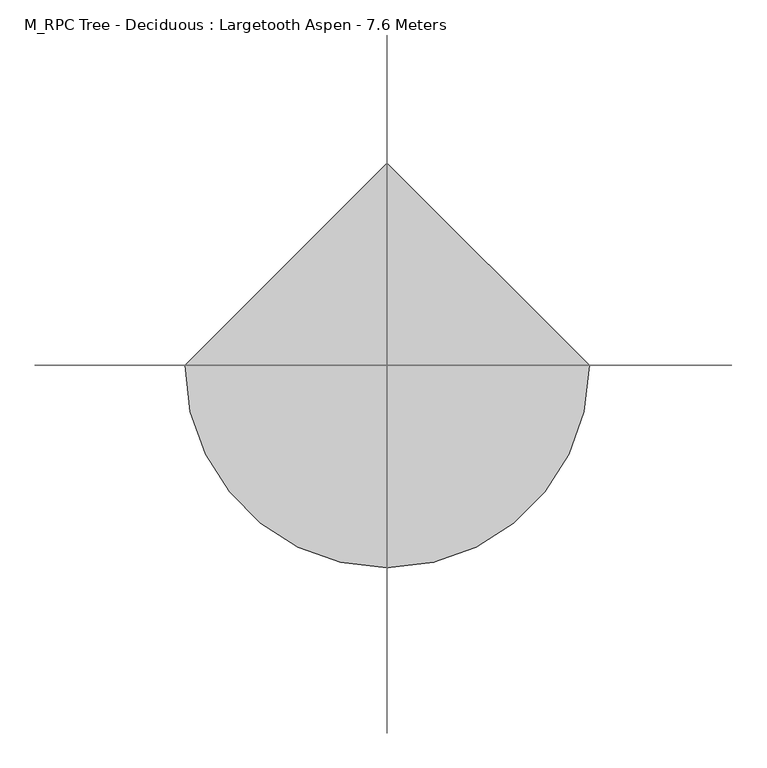
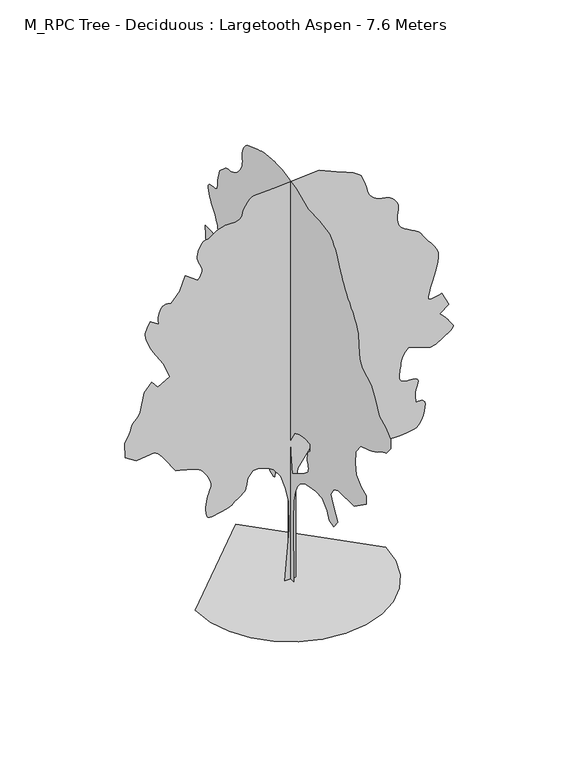
"""IFC4 building model written with IfcOpenShell, lengths in millimetres: geographic element geometry, M_RPC Tree - Deciduous : Largetooth Aspen - 7.6 Meters."""

import ifcopenshell
import ifcopenshell.guid

model = None  # the IFC model being written
_history = None  # IfcOwnerHistory: only IFC2X3 demands one
_inside = {}  # id of a spatial element -> (the spatial element, [elements in it])
_under = {}  # id of a project, library or spatial element -> (it, [spatial elements below it])
_declared = {}  # id of a project -> (the project, [libraries it declares])
_typed = {}  # id of a type object -> (the type object, [elements of that type])
_made_of = {}  # id of a material, layer set ... -> (it, [elements and type objects made of it])


def new_model(schema):
    """Start an empty IFC model of exactly this schema.

    Asked for "IFC4X3", IfcOpenShell would pick the latest addendum, in which some entities
    have other attributes; the version numbers below select the first issue.
    IFC2X3 requires an IfcOwnerHistory on every rooted entity: one is made here for all.
    """
    global model, _history
    if schema == "IFC4X3":
        model = ifcopenshell.file(schema_version=(4, 3, 0, 0))
    else:
        model = ifcopenshell.file(schema=schema)
    _inside.clear()
    _under.clear()
    _declared.clear()
    _typed.clear()
    _made_of.clear()
    _history = None
    if model.schema == "IFC2X3":
        org = make("IfcOrganization", Name="unknown")
        user = make(
            "IfcPersonAndOrganization",
            ThePerson=make("IfcPerson", FamilyName="unknown"),
            TheOrganization=org,
        )
        app = make(
            "IfcApplication",
            ApplicationDeveloper=org,
            Version="unknown",
            ApplicationFullName="unknown",
            ApplicationIdentifier="unknown",
        )
        _history = make(
            "IfcOwnerHistory",
            OwningUser=user,
            OwningApplication=app,
            ChangeAction="ADDED",
            CreationDate=0,
        )
    return model


def make(cls, **values):
    """One entity of the class cls with the attributes given. An attribute that is None is left unset."""
    return model.create_entity(
        cls, **{name: value for name, value in values.items() if value is not None}
    )


def rooted(cls, **values):
    """An entity with a GlobalId (a new one), such as an element, a storey or a relation."""
    return make(cls, GlobalId=ifcopenshell.guid.new(), OwnerHistory=_history, **values)


def si_unit(unit_type, name, prefix=None):
    """IfcSIUnit, for example si_unit("LENGTHUNIT", "METRE", prefix="MILLI")."""
    return make("IfcSIUnit", UnitType=unit_type, Prefix=prefix, Name=name)


def assignment(units):
    """IfcUnitAssignment: the units of a project."""
    return None if units is None else make("IfcUnitAssignment", Units=units)


def point(xyz):
    """IfcCartesianPoint."""
    return None if xyz is None else make("IfcCartesianPoint", Coordinates=xyz)


def direction(xyz):
    """IfcDirection."""
    return None if xyz is None else make("IfcDirection", DirectionRatios=xyz)


def frame(location, z_axis=None, x_axis=None):
    """IfcAxis2Placement3D, a coordinate frame: its origin and axes. An axis left out is left unset."""
    return make(
        "IfcAxis2Placement3D",
        Location=point(location),
        Axis=direction(z_axis),
        RefDirection=direction(x_axis),
    )


def origin():
    """The frame at (0, 0, 0) with its axes left unset."""
    return frame((0.0, 0.0, 0.0))


def place(relative_to, where):
    """IfcLocalPlacement: puts the frame where relative to a parent placement (None: the world)."""
    return make(
        "IfcLocalPlacement", PlacementRelTo=relative_to, RelativePlacement=where
    )


def context(
    kind, dimensions, precision=None, world=None, true_north=None, identifier=None
):
    """IfcGeometricRepresentationContext, for example the 3D "Model" context."""
    return make(
        "IfcGeometricRepresentationContext",
        ContextIdentifier=identifier,
        ContextType=kind,
        CoordinateSpaceDimension=dimensions,
        Precision=precision,
        WorldCoordinateSystem=world,
        TrueNorth=true_north,
    )


def project(units=None, contexts=None):
    """IfcProject with its units and contexts."""
    return rooted(
        "IfcProject",
        Name="project",
        RepresentationContexts=contexts,
        UnitsInContext=assignment(units),
    )


def spatial(cls, under=None, at=None, **own):
    """A site, building, storey or space (cls), placed at a placement, below another one or the project."""
    s = rooted(cls, ObjectPlacement=at, **own)
    if under is not None:
        _under.setdefault(under.id(), (under, []))[1].append(s)
    return s


def point_list(points):
    """IfcCartesianPointList2D or 3D."""
    cls = (
        "IfcCartesianPointList2D" if len(points[0]) == 2 else "IfcCartesianPointList3D"
    )
    return make(cls, CoordList=points)


def triangles(points, corners, closed=None, point_numbers=None):
    """IfcTriangulatedFaceSet: each triangle names its three corners, points numbered from 1."""
    return make(
        "IfcTriangulatedFaceSet",
        Coordinates=point_list(points),
        Closed=closed,
        CoordIndex=corners,
        PnIndex=point_numbers,
    )


def shape(context_of_items, identifier, shape_type, items):
    """IfcShapeRepresentation: the items that make up one representation, for example the "Body"."""
    return make(
        "IfcShapeRepresentation",
        ContextOfItems=context_of_items,
        RepresentationIdentifier=identifier,
        RepresentationType=shape_type,
        Items=items,
    )


def source(mapping_origin, context_of_items, identifier, shape_type, items):
    """IfcRepresentationMap: a shape defined once, which mapped items show again and again."""
    return make(
        "IfcRepresentationMap",
        MappingOrigin=mapping_origin,
        MappedRepresentation=shape(context_of_items, identifier, shape_type, items),
    )


def transform(
    local_origin,
    x_axis=None,
    y_axis=None,
    z_axis=None,
    scale=None,
    scale2=None,
    scale3=None,
    uniform=True,
):
    """IfcCartesianTransformationOperator3D, or its non-uniform kind. x_axis, y_axis, z_axis: its Axis1, 2, 3."""
    if uniform:
        return make(
            "IfcCartesianTransformationOperator3D",
            Axis1=direction(x_axis),
            Axis2=direction(y_axis),
            LocalOrigin=point(local_origin),
            Scale=scale,
            Axis3=direction(z_axis),
        )
    return make(
        "IfcCartesianTransformationOperator3DnonUniform",
        Axis1=direction(x_axis),
        Axis2=direction(y_axis),
        LocalOrigin=point(local_origin),
        Scale=scale,
        Axis3=direction(z_axis),
        Scale2=scale2,
        Scale3=scale3,
    )


def mapped(mapping_source, mapping_target):
    """IfcMappedItem: shows the shape of a source again, moved by a transform."""
    return make(
        "IfcMappedItem", MappingSource=mapping_source, MappingTarget=mapping_target
    )


def made_of(thing, what):
    """Note that an element or type object is made of a material, layer set ...; save() writes the relation."""
    if what is not None:
        _made_of.setdefault(what.id(), (what, []))[1].append(thing)
    return thing


def element(
    cls,
    number,
    at=None,
    inside=None,
    cuts=None,
    type_object=None,
    material=None,
    context=None,
    identifier="Body",
    shape_type=None,
    held_by="IfcProductDefinitionShape",
    body=None,
    shapes=None,
    **own,
):
    """One element of the class cls, such as IfcWall. Its Tag is "e" and its number.

    at: its placement. inside: the storey or other place that contains it. cuts: it is an
    opening in that element (IfcRelVoidsElement). A single representation is given by context,
    identifier, shape_type and body (its items); several are given by shapes. held_by: the class
    of the entity that holds the representations. save() writes the other relations.
    """
    e = rooted(cls, Tag="e%d" % number, ObjectPlacement=at, **own)
    if body is not None:
        shapes = [shape(context, identifier, shape_type, body)]
    if shapes is not None:
        e.Representation = make(held_by, Representations=shapes)
    if inside is not None:
        _inside.setdefault(inside.id(), (inside, []))[1].append(e)
    if cuts is not None:
        rooted(
            "IfcRelVoidsElement", RelatingBuildingElement=cuts, RelatedOpeningElement=e
        )
    if type_object is not None:
        _typed.setdefault(type_object.id(), (type_object, []))[1].append(e)
    return made_of(e, material)


def aggregate(whole, parts):
    """IfcRelAggregates: a whole, such as a stair, and the parts it consists of."""
    return rooted("IfcRelAggregates", RelatingObject=whole, RelatedObjects=parts)


def save(model, path):
    """Write the relations noted so far, then the file.

    IfcRelAggregates (storeys below a building ...), IfcRelContainedInSpatialStructure (elements
    in a storey), IfcRelDefinesByType, IfcRelAssociatesMaterial and IfcRelDeclares: one each for
    every whole, place, type object, material and project.
    """
    for whole, parts in _under.values():
        aggregate(whole, parts)
    for where, things in _inside.values():
        rooted(
            "IfcRelContainedInSpatialStructure",
            RelatedElements=things,
            RelatingStructure=where,
        )
    for kind, things in _typed.values():
        rooted("IfcRelDefinesByType", RelatedObjects=things, RelatingType=kind)
    for what, things in _made_of.values():
        rooted("IfcRelAssociatesMaterial", RelatedObjects=things, RelatingMaterial=what)
    for by, libraries in _declared.values():
        rooted("IfcRelDeclares", RelatingContext=by, RelatedDefinitions=libraries)
    model.write(path)


def m_rpc_tree_deciduous_largetooth_aspen_7_6_meters_7a32e79d(model_context):
    return source(origin(), model_context, "Body", "Tessellation", [
        triangles([(92.8617737, 0.000406, 0.005513), (-103.915959, 0.000406, 0.005513), (-22.8901635, 0.0003494, 949.168154), (-34.4652064, 0.0003176, 1481.626133), (-92.3406663, 0.0003011, 1759.4311237), (-173.3674883, 0.0002866, 2002.5093098), (-300.6937099, 0.0002762, 2176.1362118), (-404.8693279, 0.0002728, 2234.0127663), (-566.9214277, 0.0002694, 2291.8891754), (-682.6743914, 0.0002694, 2291.8891754), (-763.7004776, 0.0002762, 2176.1362118), (-798.427355, 0.0002852, 2025.6589142), (-801.2950579, 0.0002863, 2008.1460297), (-806.4934324, 0.0002874, 1989.7185207), (-816.3455927, 0.0002886, 1969.4722275), (-833.1871519, 0.0002899, 1946.489764), (-859.3387533, 0.0002915, 1919.8644997), (-897.1360102, 0.0002934, 1888.6816647), (-948.9046526, 0.0002956, 1852.0320122), (-998.3097038, 0.0002977, 1817.003627), (-1032.3247061, 0.0002993, 1790.0718407), (-1058.2431822, 0.0003005, 1769.4200489), (-1083.3510246, 0.0003015, 1753.2220551), (-1114.9365967, 0.0003023, 1739.6560226), (-1160.2933485, 0.000303, 1726.8980804), (-1226.7072453, 0.0003038, 1713.1294441), (-1299.8367931, 0.0003048, 1697.5064152), (-1361.0192505, 0.0003056, 1683.0943588), (-1411.0653236, 0.0003062, 1673.9516029), (-1450.7854282, 0.0003062, 1674.1187439), (-1480.9902706, 0.0003054, 1687.6517841), (-1502.4856155, 0.0003035, 1718.5964069), (-1516.0869656, 0.0003004, 1771.0059986), (-1522.0251205, 0.0002967, 1833.4045155), (-1521.0802654, 0.0002932, 1891.7521168), (-1514.8710514, 0.00029, 1946.2541679), (-1505.0164204, 0.0002869, 1997.1108021), (-1493.1376396, 0.0002841, 2044.5246231), (-1480.8535057, 0.0002815, 2088.6983803), (-1469.7852859, 0.000279, 2129.8371483), (-1458.1775642, 0.0002769, 2165.8103886), (-1444.9485752, 0.000275, 2196.5194153), (-1432.7328964, 0.0002733, 2225.2042923), (-1424.1600185, 0.0002715, 2255.1052288), (-1421.8648098, 0.0002695, 2289.4596725), (-1428.479377, 0.000267, 2331.5079781), (-1446.6358269, 0.0002638, 2384.4900639), (-1473.3978561, 0.0002604, 2441.7913628), (-1503.3976238, 0.0002573, 2494.2338013), (-1535.6266159, 0.0002545, 2541.2094223), (-1569.0690514, 0.0002521, 2582.1229134), (-1602.7142361, 0.00025, 2616.3228607), (-1635.5487144, 0.0002484, 2643.2520309), (-1666.5644085, 0.0002473, 2662.3026123), (-1701.7269424, 0.0002464, 2677.1732162), (-1746.6125748, 0.0002455, 2692.0694), (-1799.5946606, 0.0002446, 2706.940004), (-1859.0570194, 0.0002437, 2721.8358971), (-1923.3782387, 0.0002428, 2736.706501), (-1990.9396671, 0.000242, 2751.5773956), (-2060.1198921, 0.0002411, 2766.4732887), (-2256.8962532, 0.0002238, 3055.8556252), (-2301.7818855, 0.0002202, 3116.5289566), (-2338.160479, 0.0002175, 3161.4195305), (-2367.4508423, 0.0002156, 3193.1367805), (-2391.0741096, 0.0002144, 3214.3154297), (-2410.4440029, 0.0002136, 3227.61549), (-2426.9816563, 0.0002131, 3235.6461044), (-2442.1006462, 0.0002128, 3241.041996), (-2766.1945267, 0.0002148, 3206.3353935), (-2962.9836777, 0.0002073, 3333.6607613), (-2974.5611687, 0.0001914, 3599.8884064), (-2952.3436295, 0.000189, 3639.5351143), (-2930.8612198, 0.0001867, 3678.9789276), (-2910.7717484, 0.0001843, 3718.0431129), (-2892.8103447, 0.0001821, 3756.473616), (-2877.7118477, 0.0001798, 3794.0937035), (-2866.1343567, 0.0001776, 3830.70019), (-2858.8132919, 0.0001755, 3866.1160515), (-2847.3878265, 0.0001735, 3899.5814507), (-2825.6772331, 0.0001716, 3931.2481224), (-2797.4559906, 0.0001698, 3962.0787987), (-2766.6000252, 0.0001679, 3993.137368), (-2736.9852631, 0.000166, 4025.3865623), (-2712.4120537, 0.000164, 4059.8905609), (-2696.7560326, 0.0001617, 4097.611805), (-2627.2919586, 0.000141, 4444.881015), (-2488.4021805, 0.0001321, 4595.3354942), (-2384.2240917, 0.0001396, 4468.0101265), (-2164.2955101, 0.0001327, 4583.7835831), (-2280.0484737, 0.0001155, 4873.1406303), (-2465.2501053, 9.82e-05, 5162.5226761), (-2487.5231644, 9.58e-05, 5203.6643509), (-2513.0364326, 9.27e-05, 5254.9385468), (-2539.3601166, 8.93e-05, 5312.268187), (-2564.0600624, 8.58e-05, 5371.6238663), (-2584.7067673, 8.24e-05, 5428.9535065), (-2598.8934013, 7.93e-05, 5480.2277023), (-2604.1628471, 7.69e-05, 5521.3693771), (-2601.4519661, 7.48e-05, 5555.7463486), (-2593.9027176, 7.28e-05, 5589.5413788), (-2582.2746483, 7.08e-05, 5622.8038834), (-2567.4293335, 6.89e-05, 5655.6611801), (-2550.1521904, 6.69e-05, 5688.2394241), (-2531.2585762, 6.5e-05, 5720.5903564), (-2511.5516396, 6.31e-05, 5752.8651306), (-2361.0744873, 6.93e-05, 5648.6941635), (-2365.8675087, 6.73e-05, 5681.019516), (-2369.6472198, 6.54e-05, 5713.8518143), (-2371.4003105, 6.34e-05, 5747.6968414), (-2370.118412, 6.13e-05, 5783.0621246), (-2364.7857433, 5.9e-05, 5820.4540283), (-2354.391465, 5.67e-05, 5860.3794983), (-2337.9248829, 5.41e-05, 5903.344899), (-2316.394075, 5.19e-05, 5940.9141174), (-2291.8258072, 5.04e-05, 5965.7155106), (-2264.7268799, 4.95e-05, 5979.8768555), (-2235.6036575, 4.92e-05, 5985.5515091), (-2204.9604698, 4.92e-05, 5984.8422501), (-2173.3064426, 4.95e-05, 5979.8768555), (-2141.1459057, 5e-05, 5972.7836838), (-1990.6686081, 3.96e-05, 6146.4178528), (-1886.4929901, 2.44e-05, 6401.0685883), (-1666.5644085, 3.41e-05, 6239.0110382), (-1644.4939533, 3.23e-05, 6268.8284042), (-1623.9409927, 3.05e-05, 6298.823085), (-1606.4256374, 2.87e-05, 6329.2229736), (-1593.4675621, 2.69e-05, 6360.2309647), (-1586.584552, 2.5e-05, 6392.0749512), (-1587.2913403, 2.3e-05, 6424.9066681), (-1597.1131245, 2.1e-05, 6458.9551712), (-1613.1085144, 1.89e-05, 6493.7885101), (-1630.1173599, 1.68e-05, 6529.2043716), (-1646.3154991, 1.46e-05, 6565.8614365), (-1659.8813862, 1.23e-05, 6604.3428085), (-1668.993766, 9.9e-06, 6645.2310104), (-1671.8286221, 7.3e-06, 6689.1585617), (-1666.5644085, 4.4e-06, 6736.759726), (-1653.9432312, 1.5e-06, 6785.3747818), (-1636.4607227, -1.2e-06, 6830.974324), (-1614.9300602, -3.6e-06, 6871.9131042), (-1590.1616592, -5.7e-06, 6906.5691284), (-1562.9612846, -7.3e-06, 6933.3209839), (-1534.1394974, -8.3e-06, 6950.5728378), (-1504.512236, -8.7e-06, 6956.6782791), (-1471.3382435, -9.2e-06, 6965.0132355), (-1431.8891979, -1.05e-05, 6986.521225), (-1386.9707188, -1.22e-05, 7015.9078033), (-1337.3959831, -1.41e-05, 7047.9291046), (-1283.9756973, -1.59e-05, 7077.315683), (-1227.5178062, -1.72e-05, 7098.8236725), (-1168.8306908, -1.77e-05, 7107.1580475), (-1109.0314339, -1.76e-05, 7106.8289978), (-1050.4481638, -1.77e-05, 7107.2847839), (-995.7104439, -1.79e-05, 7110.8060806), (-947.4530697, -1.84e-05, 7119.5718246), (-908.3055319, -1.94e-05, 7135.8353668), (-880.9024807, -2.09e-05, 7161.8273849), (-867.8760956, -2.32e-05, 7199.7512329), (-856.9422426, -2.61e-05, 7248.5941818), (-835.6824938, -2.93e-05, 7302.6809967), (-806.5264246, -3.26e-05, 7357.4009125), (-771.9008492, -3.56e-05, 7408.0420074), (-734.2403572, -3.81e-05, 7449.9940979), (-695.9718355, -3.98e-05, 7478.5696793), (-659.5247869, -4.04e-05, 7489.1341507), (-323.8458215, -4.18e-05, 7512.2885513), (509.5693688, -4.53e-05, 7570.1751343), (926.2744205, -3.42e-05, 7384.9631836), (995.3532709, -3.26e-05, 7357.5526474), (1062.2079111, -3.09e-05, 7329.4578506), (1124.6038118, -2.92e-05, 7299.9195374), (1180.3219225, -2.73e-05, 7268.2778641), (1227.1277138, -2.52e-05, 7233.7741562), (1262.7970482, -2.29e-05, 7195.7485703), (1285.1055702, -2.04e-05, 7153.4674301), (1299.9533558, -1.79e-05, 7111.9461273), (1314.5985374, -1.58e-05, 7075.1117477), (1328.8409821, -1.37e-05, 7040.4813034), (1342.4753242, -1.16e-05, 7005.6479645), (1355.2991055, -9.4e-06, 6968.1799026), (1367.1094311, -6.8e-06, 6925.6702881), (1377.7063133, -3.9e-06, 6875.662294), (1393.5345623, -8e-07, 6823.9573105), (1419.2834267, 2e-06, 6778.1292938), (1452.117905, 4.3e-06, 6738.3811386), (1489.2059029, 6.3e-06, 6704.890741), (1527.709948, 7.9e-06, 6677.9109924), (1564.7979458, 9.1e-06, 6657.5936279), (1597.6348949, 9.9e-06, 6644.1415421), (1628.0070236, 1.04e-05, 6636.0856384), (1659.1872425, 1.07e-05, 6630.6638763), (1690.5726814, 1.1e-05, 6626.2310074), (1721.5527672, 1.13e-05, 6621.2150345), (1751.5195427, 1.17e-05, 6613.9439667), (1779.8675217, 1.24e-05, 6602.8481323), (1805.9862762, 1.34e-05, 6586.2799576), (1831.2638031, 1.47e-05, 6563.7586578), (1856.5388592, 1.63e-05, 6536.6015945), (1880.3977226, 1.82e-05, 6505.7964981), (1901.4218754, 2.02e-05, 6472.3560974), (1918.1949795, 2.23e-05, 6437.2948654), (1929.2986622, 2.44e-05, 6401.625531), (1933.3139694, 2.65e-05, 6366.3364059), (1929.8053173, 2.9e-05, 6325.1191544), (1922.245895, 3.2e-05, 6273.1351181), (1915.0916805, 3.56e-05, 6213.8805954), (1912.7964718, 3.93e-05, 6150.775145), (1919.8163921, 4.31e-05, 6087.2644867), (1940.6048035, 4.67e-05, 6026.7937592), (1979.615649, 5e-05, 5972.7836838), (2034.2165314, 5.26e-05, 5927.5631882), (2096.1082478, 5.5e-05, 5888.8289246), (2161.2403187, 5.71e-05, 5853.1340103), (2225.5615379, 5.92e-05, 5817.0088898), (2285.0238968, 6.16e-05, 5777.0584213), (2335.5764797, 6.44e-05, 5729.8118866), (2373.1711327, 6.79e-05, 5671.8491455), (2411.6423309, 7.17e-05, 5607.2240204), (2462.6659607, 7.56e-05, 5541.7878983), (2518.9567108, 7.96e-05, 5474.7303635), (2573.2307236, 8.38e-05, 5405.2415817), (2618.1721664, 8.81e-05, 5332.5093933), (2646.5201454, 9.27e-05, 5255.7495438), (2650.9785942, 9.76e-05, 5174.1004578), (2634.6386032, 0.0001032, 5079.7841217), (2608.190799, 0.0001097, 4970.8762344), (2575.6628426, 0.0001165, 4855.508567), (2541.0826859, 0.0001233, 4741.7367325), (2508.5625778, 0.0001295, 4637.6927925), (2482.1043091, 0.0001347, 4551.4835197), (2465.7718758, 0.0001383, 4491.1648178), (2464.9611694, 0.0001404, 4454.9635391), (2480.5538223, 0.0001417, 4433.9369156), (2509.8113388, 0.0001422, 4425.5769608), (2550.0001648, 0.0001421, 4427.3248192), (2598.3867462, 0.0001415, 4436.6727951), (2652.2453773, 0.0001407, 4451.0876129), (2708.839888, 0.0001396, 4468.0101265), (2836.1652557, 0.0001548, 4213.3596817), (2674.1332855, 0.0001624, 4086.0346046), (2698.8841003, 0.0001637, 4063.6400414), (2723.4573097, 0.0001651, 4040.7132431), (2747.6253113, 0.0001665, 4016.7987144), (2771.1852104, 0.0001681, 3991.3386406), (2793.9346939, 0.0001697, 3963.8775261), (2815.6705765, 0.0001715, 3933.8828453), (2836.1652557, 0.0001735, 3900.8482338), (2858.1037422, 0.0001754, 3868.6749069), (2881.2584335, 0.000177, 3840.554821), (2901.1705902, 0.0001786, 3814.8921432), (2913.3811821, 0.0001801, 3790.0148827), (2913.4570496, 0.0001816, 3764.3269157), (2896.9144547, 0.0001833, 3736.2324097), (2859.3199471, 0.0001852, 3704.0590828), (2604.6695023, 0.0001955, 3530.4246231), (2500.4962097, 0.0001962, 3518.8471321), (2118.5182171, 0.0001886, 3646.1724998), (2091.3836815, 0.0001903, 3618.7110947), (2065.163625, 0.000192, 3590.1352226), (2040.7651142, 0.0001938, 3559.3298355), (2019.0975414, 0.0001958, 3525.1551773), (2001.0780018, 0.0001981, 3486.5726486), (1987.6134167, 0.0002008, 3442.3913338), (1979.615649, 0.0002038, 3391.5220551), (1974.0473843, 0.0002068, 3342.1474525), (1967.6684132, 0.0002092, 3301.2848305), (1961.0868382, 0.0002113, 3266.096862), (1954.9106163, 0.0002132, 3233.7209312), (1949.7477047, 0.0002151, 3201.3702896), (1946.2035896, 0.0002172, 3166.1567413), (1944.888699, 0.0002197, 3125.2941193), (1953.8643139, 0.000222, 3086.7368797), (1977.0163891, 0.0002236, 3059.0981598), (2008.6704163, 0.0002247, 3040.5542336), (2043.1591541, 0.0002254, 3029.3316628), (2074.8131813, 0.0002257, 3023.5555618), (2097.9652565, 0.0002259, 3021.4277847), (2106.9408714, 0.0002259, 3021.1237335), (2119.5973663, 0.0002258, 3022.0103073), (2151.4869896, 0.0002258, 3022.4663841), (2193.5021576, 0.000226, 3019.2997169), (2236.5307812, 0.0002266, 3009.242482), (2271.4578644, 0.0002278, 2989.0771431), (2289.1759689, 0.0002298, 2955.5102966), (2280.5702442, 0.0002328, 2905.3758568), (2259.8146797, 0.0002362, 2847.8691925), (2246.3500946, 0.0002394, 2794.0105614), (2238.9578133, 0.0002425, 2743.191861), (2236.4270084, 0.0002453, 2694.7799904), (2237.5416206, 0.0002481, 2648.2174255), (2241.0857357, 0.0002508, 2602.8707748), (2245.8434395, 0.0002535, 2558.1069374), (2285.1910378, 0.0002532, 2562.540097), (2322.5171024, 0.0002531, 2563.730722), (2355.7899261, 0.0002535, 2558.4106979), (2382.9903008, 0.0002544, 2543.4133575), (2402.0916058, 0.000256, 2515.4278564), (2411.0672207, 0.0002587, 2471.2540993), (2407.8954666, 0.0002625, 2407.6396683), (2395.1731327, 0.0002668, 2334.9507912), (2376.983836, 0.0002708, 2266.9155544), (2353.5301804, 0.0002745, 2205.3632069), (2325.0124443, 0.0002777, 2152.110062), (2291.638464, 0.0002803, 2108.9801365), (2253.6054657, 0.0002821, 2077.7999176), (2211.1189602, 0.0002832, 2060.3858643), (2171.2620907, 0.0002837, 2051.7801395), (2137.4826118, 0.000284, 2045.4011684), (2104.5113686, 0.0002843, 2040.64361), (2067.0864727, 0.0002845, 2036.8967457), (2019.9412399, 0.0002847, 2033.5578506), (1957.8137821, 0.000285, 2030.0137356), (1875.4374149, 0.0002852, 2025.6589142), (1785.9069786, 0.0002851, 2027.1105698), (1704.880965, 0.0002844, 2040.1039627), (1630.9407108, 0.000283, 2062.7139198), (1562.6724941, 0.0002812, 2093.0175934), (1498.6551807, 0.0002791, 2129.0947517), (1437.4727234, 0.0002767, 2169.0176056), (1377.7063133, 0.0002742, 2210.8631618), (1123.0508543, 0.0002597, 2453.9412025), (856.8231365, 0.0002528, 2569.6841377), (544.2937391, 0.0002542, 2546.5547356), (393.8164052, 0.0002611, 2430.7917435), (289.6407872, 0.00027, 2280.3144459), (127.5871523, 0.0002838, 2048.8109894), (92.8617737, 0.0003011, 1759.4311237), (92.8617737, 0.0003383, 1134.3723289), (-0.0023646, 90.6053344, 1.1e-05), (-0.0023646, -94.5971056, 0.0), (-0.0023646, -83.0220672, 1157.5168465), (-0.0023646, -94.5971056, 1527.9227257), (-0.0023646, -140.8980313, 1724.6992321), (-0.0023646, -210.3490428, 1875.1765297), (-0.0023646, -302.9508941, 1990.9294933), (-0.0023646, -441.853444, 2071.9555069), (-0.0023646, -557.6038642, 2095.1051113), (-0.0023646, -789.1072117, 2141.4067909), (-0.0023646, -985.8861889, 2129.8320614), (-0.0023646, -1136.3635592, 1979.3547638), (-0.0023646, -1205.8147705, 1840.4521957), (-0.0023646, -1333.1399929, 1794.1505161), (-0.0023646, -1472.042561, 1967.7774181), (-0.0023646, -1321.5652634, 2199.2833454), (-0.0023646, -1252.1139793, 2361.3353725), (-0.0023646, -1333.1399929, 2500.2354698), (-0.0023646, -1483.6172905, 2569.6841377), (-0.0023646, -1969.7736626, 2569.6841377), (-0.0023646, -2351.7542713, 2835.9117828), (-0.0023646, -2351.7542713, 2997.9690422), (-0.0023646, -2189.7022442, 3067.4075363), (-0.0023646, -2039.2249466, 3206.3101044), (-0.0023646, -2004.5006126, 3403.0992554), (-0.0023646, -2027.6500717, 3634.5950089), (-0.0023646, -2178.1273693, 3831.3841599), (-0.0023646, -2444.3551598, 3923.9773453), (-0.0023646, -2488.9367409, 3941.4068047), (-0.0023646, -2533.110498, 3959.1147354), (-0.0023646, -2576.4735489, 3977.4307686), (-0.0023646, -2618.6279526, 3996.6839539), (-0.0023646, -2659.1612343, 4017.1280548), (-0.0023646, -2697.6678955, 4039.0921211), (-0.0023646, -2733.7427284, 4062.8799133), (-0.0023646, -2768.4493309, 4086.3386559), (-0.0023646, -2803.1812225, 4107.3652794), (-0.0023646, -2837.9131142, 4126.3652824), (-0.0023646, -2872.6450058, 4143.7438728), (-0.0023646, -2907.351899, 4159.9065491), (-0.0023646, -2942.0837906, 4175.258519), (-0.0023646, -2976.8156822, 4190.2052811), (-0.0023646, -3104.14105, 4352.2622498), (-0.0023646, -3104.14105, 4514.3195091), (-0.0023646, -2953.6609909, 4653.2220772), (-0.0023646, -2756.8971291, 4757.3927536), (-0.0023646, -2629.5467628, 5000.4657074), (-0.0023646, -2502.234185, 5185.6776581), (-0.0023646, -2224.4291943, 5336.1574265), (-0.0023646, -2143.4030354, 5463.4827942), (-0.0023646, -2120.2509602, 5718.1329483), (-0.0023646, -2097.1013557, 5926.4743011), (-0.0023646, -2072.264645, 5978.4327576), (-0.0023646, -2047.225185, 6029.4540619), (-0.0023646, -2021.7779011, 6078.651059), (-0.0023646, -1995.7251308, 6125.1127579), (-0.0023646, -1968.8641251, 6167.9514221), (-0.0023646, -1940.9873383, 6206.2043198), (-0.0023646, -1911.8997242, 6239.0110382), (-0.0023646, -1875.8225658, 6277.7964615), (-0.0023646, -1830.2327614, 6330.9455429), (-0.0023646, -1779.7788643, 6393.0121033), (-0.0023646, -1729.1274502, 6458.4988037), (-0.0023646, -1682.9270725, 6521.9844635), (-0.0023646, -1645.83922, 6577.9705811), (-0.0023646, -1622.5198586, 6620.9865601), (-0.0023646, -1605.6807701, 6657.1372604), (-0.0023646, -1585.6016178, 6696.1255783), (-0.0023646, -1563.2930958, 6737.9253525), (-0.0023646, -1539.7736012, 6782.5877426), (-0.0023646, -1516.0490318, 6830.0627518), (-0.0023646, -1493.1350235, 6880.3742157), (-0.0023646, -1472.042561, 6933.5238785), (-0.0023646, -1448.8245014, 6986.749118), (-0.0023646, -1419.5316673, 7037.5425293), (-0.0023646, -1385.1772236, 7086.3087387), (-0.0023646, -1346.7743351, 7133.4541168), (-0.0023646, -1305.3316612, 7179.3832901), (-0.0023646, -1261.8673084, 7224.5020477), (-0.0023646, -1217.3895727, 7269.2155975), (-0.0023646, -893.2828297, 7327.0766006), (-0.0023646, -546.029062, 7338.653801), (-0.0023646, -175.623419, 7500.711351), (-0.0023646, 264.2314734, 7593.3045364), (-0.0023646, 323.6937959, 7595.7363647), (-0.0023646, 382.7508379, 7597.8647232), (-0.0023646, 440.9996807, 7599.3843979), (-0.0023646, 498.0300296, 7599.9925003), (-0.0023646, 553.4441254, 7599.3843979), (-0.0023646, 606.831528, 7597.2566208), (-0.0023646, 657.7895004, 7593.3045364), (-0.0023646, 706.7891985, 7588.2379852), (-0.0023646, 754.9781902, 7582.5883301), (-0.0023646, 802.9670488, 7575.698053), (-0.0023646, 851.3612606, 7566.9828873), (-0.0023646, 900.7663118, 7555.8620544), (-0.0023646, 951.7900869, 7541.6751297), (-0.0023646, 1005.0433044, 7523.8657516), (-0.0023646, 1340.7248497, 7408.1181656), (-0.0023646, 1370.3545818, 7383.1138779), (-0.0023646, 1399.173753, 7356.8689682), (-0.0023646, 1426.3741276, 7328.2166473), (-0.0023646, 1451.1425285, 7295.9418732), (-0.0023646, 1472.6733364, 7258.7778625), (-0.0023646, 1490.1558449, 7215.5595703), (-0.0023646, 1502.7768768, 7165.019632), (-0.0023646, 1507.1292274, 7116.7342072), (-0.0023646, 1503.5851124, 7077.7714691), (-0.0023646, 1497.0060081, 7043.2421814), (-0.0023646, 1492.2458336, 7008.3076859), (-0.0023646, 1494.1711521, 6968.1293243), (-0.0023646, 1507.6358826, 6917.7916992), (-0.0023646, 1537.5012108, 6852.5078934), (-0.0023646, 1578.4019119, 6786.1851974), (-0.0023646, 1620.9238804, 6734.4546341), (-0.0023646, 1663.8485859, 6694.8587952), (-0.0023646, 1705.9652012, 6664.9908508), (-0.0023646, 1746.0576668, 6642.4189728), (-0.0023646, 1782.9075977, 6624.7107513), (-0.0023646, 1815.3063469, 6609.4093597), (-0.0023646, 1845.0703732, 6598.3135254), (-0.0023646, 1874.8345448, 6592.8923447), (-0.0023646, 1904.598571, 6590.2826202), (-0.0023646, 1934.3652134, 6587.699057), (-0.0023646, 1964.129385, 6582.2522964), (-0.0023646, 1993.8935566, 6571.1558807), (-0.0023646, 2023.6575829, 6551.5483566), (-0.0023646, 2197.2869556, 6401.0685883), (-0.0023646, 2266.7357689, 6181.1500351), (-0.0023646, 2264.4760231, 6146.5445892), (-0.0023646, 2263.5310226, 6112.7751389), (-0.0023646, 2265.2182743, 6080.6021027), (-0.0023646, 2270.8549942, 6050.8858932), (-0.0023646, 2281.7533115, 6024.3875107), (-0.0023646, 2299.23582, 6001.9417877), (-0.0023646, 2324.612178, 5984.3608841), (-0.0023646, 2359.9116222, 5974.3033585), (-0.0023646, 2402.9047829, 5970.5285889), (-0.0023646, 2448.5301956, 5967.9700241), (-0.0023646, 2491.7284309, 5961.5605316), (-0.0023646, 2527.4306122, 5946.2341415), (-0.0023646, 2550.5826874, 5916.9237213), (-0.0023646, 2556.1056061, 5868.6127167), (-0.0023646, 2547.4416, 5812.448703), (-0.0023646, 2532.0896301, 5762.3651321), (-0.0023646, 2511.1641632, 5717.3475311), (-0.0023646, 2485.7878052, 5676.3837524), (-0.0023646, 2457.0700813, 5638.4599045), (-0.0023646, 2426.1228424, 5602.562677), (-0.0023646, 2394.0634621, 5567.6531799), (-0.0023646, 2369.3610455, 5525.4987762), (-0.0023646, 2345.2664406, 5483.4705276), (-0.0023646, 2322.3854244, 5441.6201752), (-0.0023646, 2301.3284248, 5400.0732925), (-0.0023646, 2282.698312, 5358.9321991), (-0.0023646, 2267.1081299, 5318.2974701), (-0.0023646, 2255.160894, 5278.2708435), (-0.0023646, 2248.9518253, 5240.6254669), (-0.0023646, 2249.4254883, 5206.6025436), (-0.0023646, 2255.4649452, 5175.6201324), (-0.0023646, 2265.9605255, 5147.0695496), (-0.0023646, 2279.797617, 5120.3426926), (-0.0023646, 2295.861462, 5094.8320404), (-0.0023646, 2313.0374485, 5069.9294907), (-0.0023646, 2463.5147461, 5093.0844727), (-0.0023646, 2648.7240807, 5093.0844727), (-0.0023646, 2625.5693893, 4757.3927536), (-0.0023646, 2417.2130665, 4398.5716324), (-0.0023646, 2409.7574169, 4356.4422272), (-0.0023646, 2402.1979946, 4314.642453), (-0.0023646, 2394.4358231, 4273.4252014), (-0.0023646, 2386.3697456, 4233.1451019), (-0.0023646, 2377.898315, 4194.0559181), (-0.0023646, 2368.9227001, 4156.486409), (-0.0023646, 2359.3391281, 4120.7664963), (-0.0023646, 2344.9953815, 4082.1586784), (-0.0023646, 2323.9712288, 4037.2681046), (-0.0023646, 2299.5044083, 3988.3492882), (-0.0023646, 2274.8373093, 3937.5814568), (-0.0023646, 2253.2051994, 3887.2441223), (-0.0023646, 2237.8507587, 3839.5162216), (-0.0023646, 2232.0114349, 3796.6522682), (-0.0023646, 2236.7360012, 3758.6522621), (-0.0023646, 2249.9651356, 3723.6921867), (-0.0023646, 2270.279884, 3691.2656776), (-0.0023646, 2296.2641991, 3660.865789), (-0.0023646, 2326.5020336, 3631.9602859), (-0.0023646, 2359.5747242, 3604.0936729), (-0.0023646, 2394.0634621, 3576.7337151), (-0.0023646, 2706.5853745, 3646.1724998), (-0.0023646, 2723.8372284, 3596.6458717), (-0.0023646, 2740.3798233, 3547.4991623), (-0.0023646, 2755.5039001, 3499.1884483), (-0.0023646, 2768.4746201, 3452.0686501), (-0.0023646, 2778.6333023, 3406.5699738), (-0.0023646, 2785.245108, 3363.0979179), (-0.0023646, 2787.6266487, 3322.0832703), (-0.0023646, 2774.199852, 3282.9940865), (-0.0023646, 2739.6958534, 3244.7153183), (-0.0023646, 2692.8545265, 3206.6647339), (-0.0023646, 2642.3654572, 3168.1836525), (-0.0023646, 2596.9426483, 3128.7142593), (-0.0023646, 2565.3015564, 3087.5981644), (-0.0023646, 2556.1056061, 3044.2784248), (-0.0023646, 2564.4399811, 3002.6556747), (-0.0023646, 2578.8547989, 2966.5049744), (-0.0023646, 2598.3361679, 2934.9397499), (-0.0023646, 2621.8454887, 2906.9969788), (-0.0023646, 2648.4200294, 2881.7903778), (-0.0023646, 2676.9959015, 2858.3825043), (-0.0023646, 2706.5853745, 2835.9117828), (-0.0023646, 2776.0491577, 2604.4160294), (-0.0023646, 2709.3974121, 2602.1106468), (-0.0023646, 2644.6708397, 2600.945311), (-0.0023646, 2583.7949043, 2601.984201), (-0.0023646, 2528.6796638, 2606.3667824), (-0.0023646, 2481.2656975, 2615.2081032), (-0.0023646, 2443.468586, 2629.6226303), (-0.0023646, 2417.2130665, 2650.725412), (-0.0023646, 2391.9710026, 2676.8694557), (-0.0023646, 2357.0109272, 2705.4453278), (-0.0023646, 2313.9494568, 2736.0478203), (-0.0023646, 2264.407568, 2768.2973053), (-0.0023646, 2210.0068188, 2801.7371246), (-0.0023646, 2152.3684765, 2835.987941), (-0.0023646, 2093.1088669, 2870.6436745), (-0.0023646, 2090.6465172, 2833.3785072), (-0.0023646, 2088.2828533, 2795.8345779), (-0.0023646, 2086.1244095, 2757.6572571), (-0.0023646, 2084.2675461, 2718.5680733), (-0.0023646, 2082.8158905, 2678.2879738), (-0.0023646, 2081.8710354, 2636.4626198), (-0.0023646, 2081.5341373, 2592.838829), (-0.0023646, 2079.9481876, 2547.390731), (-0.0023646, 2074.514217, 2502.7332825), (-0.0023646, 2064.2212406, 2462.5418404), (-0.0023646, 2048.0560936, 2430.4471424), (-0.0023646, 2025.0077911, 2410.0995472), (-0.0023646, 1994.0631683, 2405.1366234), (-0.0023646, 1954.2062988, 2419.2093109), (-0.0023646, 1909.2219807, 2445.3635284), (-0.0023646, 1863.6321762, 2473.9469582), (-0.0023646, 1817.5331005, 2504.5546829), (-0.0023646, 1771.028817, 2536.7762627), (-0.0023646, 1724.222953, 2570.216082), (-0.0023646, 1677.2144852, 2604.4921875), (-0.0023646, 1630.1020992, 2639.147921), (-0.0023646, 1352.2995792, 2720.1639061), (-0.0023646, 1074.4945158, 2627.5707207), (-0.0023646, 900.8676138, 2419.2093109), (-0.0023646, 923.2420475, 2389.5794334), (-0.0023646, 945.9203871, 2360.7602623), (-0.0023646, 969.204213, 2333.5598877), (-0.0023646, 993.4000471, 2308.7916321), (-0.0023646, 1018.8119408, 2287.2608242), (-0.0023646, 1045.7412563, 2269.7783157), (-0.0023646, 1074.4945158, 2257.1572838), (-0.0023646, 1101.897567, 2244.8731499), (-0.0023646, 1125.0471714, 2228.3381126), (-0.0023646, 1144.6551315, 2208.258815), (-0.0023646, 1161.4257648, 2185.344952), (-0.0023646, 1176.07349, 2160.305492), (-0.0023646, 1189.3025517, 2133.8473686), (-0.0023646, 1201.8222816, 2106.6798409), (-0.0023646, 1169.4919149, 2099.1888737), (-0.0023646, 1136.6574366, 2091.3938553), (-0.0023646, 1102.8070318, 2082.9907345), (-0.0023646, 1067.4417486, 2073.6756054), (-0.0023646, 1030.0497723, 2063.1471783), (-0.0023646, 990.1269911, 2051.0986404), (-0.0023646, 947.1668226, 2037.2287022), (-0.0023646, 904.2091249, 2020.3237747), (-0.0023646, 864.2863438, 1999.7708141), (-0.0023646, 826.8943674, 1976.1830097), (-0.0023646, 791.5265408, 1950.1630863), (-0.0023646, 757.6786795, 1922.3217625), (-0.0023646, 724.8442011, 1893.2645245), (-0.0023646, 692.5138344, 1863.6018002), (-0.0023646, 692.5138344, 1701.5496277), (-0.0023646, 650.5998957, 1674.7216141), (-0.0023646, 610.2059223, 1650.6246838), (-0.0023646, 572.8469018, 1631.9970417), (-0.0023646, 540.0453429, 1621.5699165), (-0.0023646, 513.3187039, 1622.0765717), (-0.0023646, 494.1844431, 1636.2505611), (-0.0023646, 484.160055, 1666.8252937), (-0.0023646, 479.2682024, 1701.4811726), (-0.0023646, 474.7791232, 1728.6487003), (-0.0023646, 471.1007504, 1752.1706657), (-0.0023646, 468.638328, 1775.8927643), (-0.0023646, 467.7947385, 1803.6682491), (-0.0023646, 468.9752624, 1839.3374382), (-0.0023646, 472.5852528, 1886.7512592), (-0.0023646, 475.5214108, 1938.6212036), (-0.0023646, 474.812079, 1985.6298168), (-0.0023646, 471.0677945, 2028.5899853), (-0.0023646, 464.8915363, 2068.3100899), (-0.0023646, 456.893805, 2105.6006916), (-0.0023646, 447.6800869, 2141.2724968), (-0.0023646, 437.8608825, 2176.1311249), (-0.0023646, 241.0823958, 2187.7059998), (-0.0023646, 136.90626, 1990.9294933), (-0.0023646, 79.030296, 1655.2479481), (-0.0023646, 79.030296, 1226.9681305), (-0.0023646, 79.030296, 590.3344972), (-0.0022449, -48.2969385, 2025.6538273), (-0.0022449, -1.9959556, 2396.0597065), (-0.0022449, 9.5791323, 2615.9935204), (-0.0022449, -129.3229929, 2835.9117828), (-0.0022449, -279.801326, 2905.3758568), (-0.0022449, -453.4282099, 2928.5049683), (-0.0022449, -615.4803097, 2928.5049683), (-0.0022449, -615.4803097, 2789.62798), (-0.0022449, -534.4542598, 2720.1639061), (-0.0022449, -511.3046917, 2558.1069374), (-0.0022449, -521.1568156, 2548.0241226), (-0.0022449, -530.6061298, 2536.9282883), (-0.0022449, -539.2448104, 2523.7927528), (-0.0022449, -546.6699749, 2507.6277512), (-0.0022449, -552.4738358, 2487.4115433), (-0.0022449, -556.2535832, 2462.1366325), (-0.0022449, -557.6038642, 2430.7841858), (-0.0022449, -554.2294335, 2398.4207542), (-0.0022449, -544.7801193, 2370.3109875), (-0.0022449, -530.2691955, 2345.7427197), (-0.0022449, -511.7075014, 2324.0093079), (-0.0022449, -490.1108545, 2304.4038185), (-0.0022449, -466.4875508, 2286.2145218), (-0.0022449, -441.853444, 2268.7320133), (-1707.3661331, 0.0, 0.0031185), (-1662.2297894, -391.2146745, 0.0030952), (-1533.678479, -750.4840605, 0.0030738), (-1332.01012, -1067.5126745, 0.0030549), (-1067.5126745, -1332.01012, 0.0030391), (-750.4840605, -1533.678479, 0.0030271), (-391.2146745, -1662.2297894, 0.0030194), (7.48e-05, -1707.3661331, 0.0030167), (391.2146745, -1662.2297894, 0.0030194), (750.4840605, -1533.678479, 0.0030271), (1067.5126745, -1332.01012, 0.0030391), (1332.01012, -1067.5126745, 0.0030549), (1533.678479, -750.4840605, 0.0030738), (1662.2297894, -391.2146745, 0.0030952), (1707.3661331, 0.0001493, 0.0031185), (-0.0002245, 1707.3661331, 0.0032203)], [[122, 123, 124], [87, 88, 89], [1, 2, 3], [329, 1, 3], [329, 3, 4], [328, 329, 4], [328, 4, 5], [105, 106, 107], [327, 328, 5], [327, 5, 6], [104, 105, 107], [238, 239, 240], [238, 240, 241], [237, 238, 241], [236, 237, 241], [103, 104, 107], [86, 87, 89], [235, 236, 241], [102, 103, 107], [101, 102, 107], [100, 101, 107], [99, 100, 107], [98, 99, 107], [97, 98, 107], [96, 97, 107], [327, 6, 7], [326, 327, 7], [95, 96, 107], [70, 71, 72], [69, 70, 72], [69, 72, 73], [69, 73, 74], [69, 74, 75], [69, 75, 76], [69, 76, 77], [69, 77, 78], [94, 95, 107], [234, 235, 241], [93, 94, 107], [69, 78, 79], [69, 79, 80], [69, 80, 81], [69, 81, 82], [69, 82, 83], [69, 83, 84], [69, 84, 85], [68, 69, 85], [325, 326, 7], [325, 7, 8], [67, 68, 85], [92, 93, 107], [91, 92, 107], [60, 61, 62], [67, 85, 86], [67, 86, 89], [67, 89, 90], [66, 67, 90], [65, 66, 90], [64, 65, 90], [63, 64, 90], [62, 63, 90], [60, 62, 90], [59, 60, 90], [58, 59, 90], [57, 58, 90], [56, 57, 90], [55, 56, 90], [54, 55, 90], [53, 54, 90], [284, 285, 286], [283, 284, 286], [282, 283, 286], [282, 286, 287], [281, 282, 287], [280, 281, 287], [279, 280, 287], [279, 287, 288], [278, 279, 288], [277, 278, 288], [277, 288, 289], [276, 277, 289], [275, 276, 289], [275, 289, 290], [52, 53, 90], [325, 8, 9], [121, 122, 124], [275, 290, 291], [30, 31, 32], [29, 30, 32], [29, 32, 33], [28, 29, 33], [28, 33, 34], [27, 28, 34], [27, 34, 35], [27, 35, 36], [26, 27, 36], [26, 36, 37], [26, 37, 38], [25, 26, 38], [25, 38, 39], [24, 25, 39], [23, 24, 39], [22, 23, 39], [21, 22, 39], [20, 21, 39], [20, 39, 40], [20, 40, 41], [20, 41, 42], [19, 20, 42], [19, 42, 43], [18, 19, 43], [18, 43, 44], [17, 18, 44], [16, 17, 44], [15, 16, 44], [14, 15, 44], [13, 14, 44], [12, 13, 44], [11, 12, 44], [11, 44, 45], [11, 45, 46], [10, 11, 46], [10, 46, 47], [10, 47, 48], [10, 48, 49], [10, 49, 50], [10, 50, 51], [252, 253, 254], [251, 252, 254], [251, 254, 255], [250, 251, 255], [249, 250, 255], [249, 255, 256], [248, 249, 256], [247, 248, 256], [246, 247, 256], [245, 246, 256], [245, 256, 257], [245, 257, 258], [244, 245, 258], [243, 244, 258], [242, 243, 258], [241, 242, 258], [234, 241, 258], [233, 234, 258], [274, 275, 291], [324, 325, 9], [51, 52, 90], [10, 51, 90], [9, 10, 90], [324, 9, 90], [323, 324, 90], [323, 90, 91], [323, 91, 107], [323, 107, 108], [323, 108, 109], [323, 109, 110], [323, 110, 111], [323, 111, 112], [323, 112, 113], [323, 113, 114], [323, 114, 115], [323, 115, 116], [323, 116, 117], [323, 117, 118], [323, 118, 119], [323, 119, 120], [323, 120, 121], [323, 121, 124], [323, 124, 125], [323, 125, 126], [323, 126, 127], [323, 127, 128], [323, 128, 129], [322, 323, 129], [322, 129, 130], [167, 168, 169], [274, 291, 292], [296, 297, 298], [296, 298, 299], [295, 296, 299], [294, 295, 299], [294, 299, 300], [293, 294, 300], [293, 300, 301], [293, 301, 302], [293, 302, 303], [293, 303, 304], [293, 304, 305], [293, 305, 306], [293, 306, 307], [293, 307, 308], [293, 308, 309], [293, 309, 310], [293, 310, 311], [293, 311, 312], [293, 312, 313], [293, 313, 314], [293, 314, 315], [293, 315, 316], [293, 316, 317], [293, 317, 318], [293, 318, 319], [292, 293, 319], [274, 292, 319], [274, 319, 320], [274, 320, 321], [274, 321, 322], [273, 274, 322], [273, 322, 130], [272, 273, 130], [271, 272, 130], [270, 271, 130], [269, 270, 130], [268, 269, 130], [267, 268, 130], [266, 267, 130], [265, 266, 130], [264, 265, 130], [263, 264, 130], [262, 263, 130], [261, 262, 130], [260, 261, 130], [259, 260, 130], [258, 259, 130], [233, 258, 130], [232, 233, 130], [231, 232, 130], [230, 231, 130], [229, 230, 130], [228, 229, 130], [227, 228, 130], [226, 227, 130], [225, 226, 130], [224, 225, 130], [223, 224, 130], [222, 223, 130], [221, 222, 130], [220, 221, 130], [219, 220, 130], [218, 219, 130], [217, 218, 130], [216, 217, 130], [215, 216, 130], [214, 215, 130], [213, 214, 130], [212, 213, 130], [211, 212, 130], [210, 211, 130], [209, 210, 130], [208, 209, 130], [207, 208, 130], [206, 207, 130], [205, 206, 130], [204, 205, 130], [203, 204, 130], [202, 203, 130], [201, 202, 130], [200, 201, 130], [199, 200, 130], [198, 199, 130], [197, 198, 130], [196, 197, 130], [195, 196, 130], [194, 195, 130], [193, 194, 130], [192, 193, 130], [191, 192, 130], [190, 191, 130], [189, 190, 130], [188, 189, 130], [187, 188, 130], [186, 187, 130], [185, 186, 130], [184, 185, 130], [183, 184, 130], [182, 183, 130], [181, 182, 130], [180, 181, 130], [179, 180, 130], [178, 179, 130], [177, 178, 130], [176, 177, 130], [175, 176, 130], [174, 175, 130], [173, 174, 130], [172, 173, 130], [171, 172, 130], [170, 171, 130], [169, 170, 130], [167, 169, 130], [167, 130, 131], [167, 131, 132], [167, 132, 133], [167, 133, 134], [167, 134, 135], [167, 135, 136], [164, 165, 166], [164, 166, 167], [163, 164, 167], [162, 163, 167], [161, 162, 167], [160, 161, 167], [159, 160, 167], [158, 159, 167], [143, 144, 145], [142, 143, 145], [141, 142, 145], [140, 141, 145], [140, 145, 146], [139, 140, 146], [138, 139, 146], [137, 138, 146], [136, 137, 146], [136, 146, 147], [136, 147, 148], [136, 148, 149], [136, 149, 150], [136, 150, 151], [136, 151, 152], [136, 152, 153], [136, 153, 154], [136, 154, 155], [136, 155, 156], [157, 158, 167], [157, 167, 136], [157, 136, 156], [634, 330, 635], [633, 634, 635], [632, 633, 635], [631, 632, 635], [540, 541, 542], [592, 593, 594], [494, 495, 496], [635, 330, 331], [635, 331, 332], [635, 332, 333], [635, 333, 334], [635, 334, 335], [658, 635, 335], [658, 335, 336], [658, 336, 337], [658, 337, 338], [540, 542, 543], [657, 658, 338], [631, 635, 636], [630, 631, 636], [518, 519, 520], [656, 657, 338], [656, 338, 339], [655, 656, 339], [654, 655, 339], [653, 654, 339], [540, 543, 544], [539, 540, 544], [518, 520, 521], [539, 544, 545], [538, 539, 545], [538, 545, 546], [538, 546, 547], [538, 547, 548], [537, 538, 548], [537, 548, 549], [536, 537, 549], [536, 549, 550], [536, 550, 551], [535, 536, 551], [535, 551, 552], [534, 535, 552], [493, 494, 496], [493, 496, 497], [343, 344, 345], [342, 343, 345], [341, 342, 345], [340, 341, 345], [340, 345, 346], [534, 552, 553], [533, 534, 553], [518, 521, 522], [350, 351, 352], [349, 350, 352], [349, 352, 353], [348, 349, 353], [533, 553, 554], [652, 653, 339], [518, 522, 523], [518, 523, 524], [533, 554, 555], [532, 533, 555], [518, 524, 525], [518, 525, 526], [518, 526, 527], [518, 527, 528], [518, 528, 529], [518, 529, 530], [518, 530, 531], [518, 531, 532], [518, 532, 555], [517, 518, 555], [516, 517, 555], [515, 516, 555], [607, 608, 609], [591, 592, 594], [591, 594, 595], [590, 591, 595], [590, 595, 596], [589, 590, 596], [588, 589, 596], [588, 596, 597], [587, 588, 597], [586, 587, 597], [586, 597, 598], [585, 586, 598], [585, 598, 599], [584, 585, 599], [584, 599, 600], [583, 584, 600], [583, 600, 601], [582, 583, 601], [514, 515, 555], [643, 644, 645], [630, 636, 637], [629, 630, 637], [581, 582, 601], [581, 601, 602], [348, 353, 354], [580, 581, 602], [580, 602, 603], [579, 580, 603], [651, 652, 339], [651, 339, 340], [651, 340, 346], [650, 651, 346], [649, 650, 346], [649, 346, 347], [648, 649, 347], [647, 648, 347], [646, 647, 347], [372, 373, 374], [371, 372, 374], [370, 371, 374], [369, 370, 374], [369, 374, 375], [368, 369, 375], [367, 368, 375], [366, 367, 375], [365, 366, 375], [364, 365, 375], [363, 364, 375], [362, 363, 375], [361, 362, 375], [360, 361, 375], [359, 360, 375], [358, 359, 375], [357, 358, 375], [356, 357, 375], [356, 375, 376], [356, 376, 377], [356, 377, 378], [645, 646, 347], [643, 645, 347], [642, 643, 347], [641, 642, 347], [641, 347, 348], [641, 348, 354], [641, 354, 355], [607, 609, 610], [513, 514, 555], [579, 603, 604], [607, 610, 611], [607, 611, 612], [607, 612, 613], [607, 613, 614], [607, 614, 615], [607, 615, 616], [607, 616, 617], [607, 617, 618], [607, 618, 619], [607, 619, 620], [607, 620, 621], [607, 621, 622], [607, 622, 623], [607, 623, 624], [606, 607, 624], [606, 624, 625], [605, 606, 625], [605, 625, 626], [604, 605, 626], [579, 604, 626], [579, 626, 627], [579, 627, 628], [579, 628, 629], [579, 629, 637], [578, 579, 637], [578, 637, 638], [355, 356, 378], [641, 355, 378], [641, 378, 379], [640, 641, 379], [639, 640, 379], [639, 379, 380], [639, 380, 381], [639, 381, 382], [639, 382, 383], [639, 383, 384], [639, 384, 385], [639, 385, 386], [639, 386, 387], [639, 387, 388], [639, 388, 389], [639, 389, 390], [639, 390, 391], [639, 391, 392], [639, 392, 393], [639, 393, 394], [639, 394, 395], [638, 639, 395], [578, 638, 395], [577, 578, 395], [577, 395, 396], [577, 396, 397], [577, 397, 398], [577, 398, 399], [577, 399, 400], [577, 400, 401], [577, 401, 402], [577, 402, 403], [577, 403, 404], [577, 404, 405], [577, 405, 406], [577, 406, 407], [577, 407, 408], [577, 408, 409], [577, 409, 410], [577, 410, 411], [577, 411, 412], [577, 412, 413], [577, 413, 414], [577, 414, 415], [577, 415, 416], [577, 416, 417], [577, 417, 418], [577, 418, 419], [577, 419, 420], [577, 420, 421], [577, 421, 422], [577, 422, 423], [577, 423, 424], [577, 424, 425], [577, 425, 426], [577, 426, 427], [577, 427, 428], [577, 428, 429], [577, 429, 430], [577, 430, 431], [577, 431, 432], [577, 432, 433], [577, 433, 434], [566, 567, 568], [566, 568, 569], [565, 566, 569], [564, 565, 569], [564, 569, 570], [563, 564, 570], [563, 570, 571], [562, 563, 571], [562, 571, 572], [561, 562, 572], [560, 561, 572], [560, 572, 573], [559, 560, 573], [559, 573, 574], [558, 559, 574], [558, 574, 575], [557, 558, 575], [556, 557, 575], [556, 575, 576], [555, 556, 576], [513, 555, 576], [513, 576, 577], [512, 513, 577], [511, 512, 577], [470, 471, 472], [469, 470, 472], [468, 469, 472], [468, 472, 473], [467, 468, 473], [467, 473, 474], [467, 474, 475], [466, 467, 475], [466, 475, 476], [466, 476, 477], [465, 466, 477], [465, 477, 478], [465, 478, 479], [464, 465, 479], [464, 479, 480], [464, 480, 481], [464, 481, 482], [463, 464, 482], [456, 457, 458], [456, 458, 459], [456, 459, 460], [510, 511, 577], [463, 482, 483], [455, 456, 460], [454, 455, 460], [453, 454, 460], [452, 453, 460], [451, 452, 460], [450, 451, 460], [450, 460, 461], [449, 450, 461], [449, 461, 462], [463, 483, 484], [492, 493, 497], [448, 449, 462], [447, 448, 462], [491, 492, 497], [462, 463, 484], [447, 462, 484], [447, 484, 485], [446, 447, 485], [446, 485, 486], [445, 446, 486], [445, 486, 487], [444, 445, 487], [444, 487, 488], [491, 497, 498], [509, 510, 577], [491, 498, 499], [491, 499, 500], [490, 491, 500], [490, 500, 501], [490, 501, 502], [490, 502, 503], [490, 503, 504], [490, 504, 505], [490, 505, 506], [490, 506, 507], [490, 507, 508], [490, 508, 509], [490, 509, 577], [489, 490, 577], [488, 489, 577], [444, 488, 577], [443, 444, 577], [442, 443, 577], [441, 442, 577], [440, 441, 577], [435, 436, 437], [434, 435, 437], [434, 437, 438], [434, 438, 439], [577, 434, 439], [440, 577, 439], [673, 674, 659], [672, 673, 659], [672, 659, 660], [671, 672, 660], [671, 660, 661], [671, 661, 662], [670, 671, 662], [669, 670, 662], [669, 662, 663], [669, 663, 664], [669, 664, 665], [669, 665, 666], [669, 666, 667], [669, 667, 668]], closed=False),
    ])


if __name__ == "__main__":
    model = new_model("IFC4")
    model_context = context("Model", 3, world=origin())
    ifc_project = project(units=[si_unit("LENGTHUNIT", "METRE", prefix="MILLI")], contexts=[model_context])
    site = spatial("IfcSite", under=ifc_project)
    building = spatial("IfcBuilding", under=site)
    placement = place(None, origin())
    m_rpc_tree_deciduous_largetooth_aspen_7_6_meters_shape = m_rpc_tree_deciduous_largetooth_aspen_7_6_meters_7a32e79d(model_context)
    element("IfcGeographicElement", 1, ObjectType="M_RPC Tree - Deciduous : Largetooth Aspen - 7.6 Meters", at=placement, inside=building, context=model_context, shape_type="MappedRepresentation", body=[
        mapped(m_rpc_tree_deciduous_largetooth_aspen_7_6_meters_shape, transform((0.0, 0.0, 0.0), x_axis=(1.0, 0.0, 0.0), y_axis=(0.0, 1.0, 0.0), z_axis=(0.0, 0.0, 1.0))),
    ])
    save(model, "model.ifc")

# Revit data of these elements
# Type "M_RPC Tree - Deciduous : Largetooth Aspen - 7.6 Meters"
#   built-in parameter 1005198 = "{2, 15},{39, RPC-16-G0VG-J3PX-MQ0P-J000-ST1L-LVER-AU},{1, 0},{1, 0},{2, 13},{1, 8},{5, Color},{1, 0},{1, 0},{3, 0.8},{3, 0.8},{3, 0.8},{1, 8},{7, BBoxMin},{1, 0},{1, 0},{1, 0},{1, 0},{1, 0},{1, 8},{7, BBoxMax},{1, 0},{1, 0},{1, 0},{1, 0},{1, 0},{2, 11},{9, RPCTypeId},{1, 0},{1, 0},{39, RPC-16-G0VG-J3PX-MQ0P-J000-ST1L-LVER-AU},{1, 6},{14, RPCPlantHeight},{1, 0},{1, 0},{7, 24.9344},{2, 11},{7, keyword},{1, 0},{1, 0},{34, :RPCs:Trees [General]:Geometry:RPC},{2, 11},{8, category},{1, 0},{1, 0},{15, Trees [General]},{2, 11},{12, LocalizedUID},{1, 0},{1, 0},{16, Largetooth Aspen},{2, 14},{6, Height},{1, 0},{1, 0},{7, 24.9344},{1, 2},{16, Cast Reflections},{1, 0},{1, 0},{1, 0},{1, 2},{12, Cast Shadows},{1, 0},{1, 0},{1, 1},{1, 2},{9, Lock View},{1, 0},{1, 0},{1, 0},{1, 4},{5, ViewC},{1, 0},{1, 0},{1, 0},{21, assetlibrary_base.fbx},{1, 5},"
#   built-in parameter 1005195 = "RPC-16-G0VG-J3PX-MQ0P-J000-ST1L-LVER-AU"
#   Type Comments = "Largetooth Aspen"
#   Height = 7.60 m
